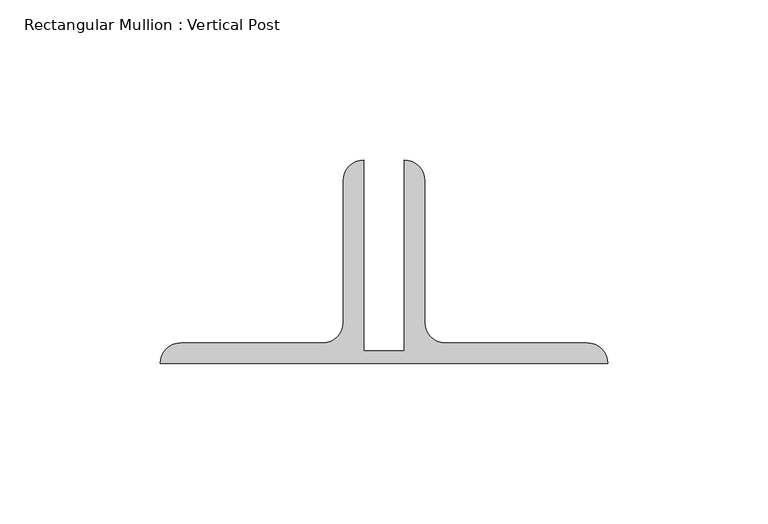
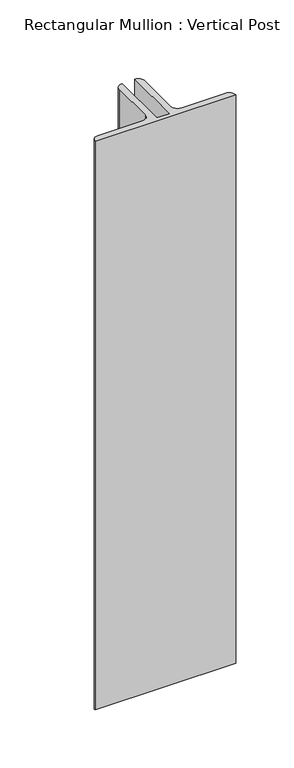
"""IFC4 building model written with IfcOpenShell, lengths in millimetres: member geometry, Rectangular Mullion : Vertical Post."""

from ifc_helpers import new_model, si_unit, point, frame, frame_2d, origin, place, context, project, spatial, polyline, circle_curve, trimmed, segment, composite_curve, outline, extrude, source, transform, mapped, element, save


def rectangular_mullion_vertical_post_30249c29(model_context):
    return source(origin(), model_context, "Body", "SweptSolid", [
        extrude(outline(composite_curve([segment(polyline([(-63.5, 22.9145205), (-63.5, 82.55)]), True, "CONTINUOUS"), segment(trimmed(circle_curve(frame_2d((-63.5, 76.2)), 6.35), [point((-63.5, 82.55))], [point((-57.15, 76.2))], False, "CARTESIAN"), True, "CONTINUOUS"), segment(polyline([(-57.15, 76.2), (-57.15, 31.75)]), True, "CONTINUOUS"), segment(trimmed(circle_curve(frame_2d((-50.8, 31.75)), 6.35), [point((-57.15, 31.75))], [point((-50.8, 25.4))], True, "CARTESIAN"), True, "CONTINUOUS"), segment(polyline([(-50.8, 25.4), (-6.35, 25.4)]), True, "CONTINUOUS"), segment(trimmed(circle_curve(frame_2d((-6.35, 19.05)), 6.35), [point((-6.35, 25.4))], [point((0.0, 19.05))], False, "CARTESIAN"), True, "CONTINUOUS"), segment(polyline([(0.0, 19.05), (-139.7, 19.05)]), True, "CONTINUOUS"), segment(trimmed(circle_curve(frame_2d((-133.35, 19.05)), 6.35), [point((-139.7, 19.05))], [point((-133.35, 25.4))], False, "CARTESIAN"), True, "CONTINUOUS"), segment(polyline([(-133.35, 25.4), (-88.9, 25.4)]), True, "CONTINUOUS"), segment(trimmed(circle_curve(frame_2d((-88.9, 31.75)), 6.35), [point((-88.9, 25.4))], [point((-82.55, 31.75))], True, "CARTESIAN"), True, "CONTINUOUS"), segment(polyline([(-82.55, 31.75), (-82.55, 76.2)]), True, "CONTINUOUS"), segment(trimmed(circle_curve(frame_2d((-76.2, 76.2)), 6.35), [point((-82.55, 76.2))], [point((-76.2, 82.55))], False, "CARTESIAN"), True, "CONTINUOUS"), segment(polyline([(-76.2, 82.55), (-76.2, 22.9145205), (-63.5, 22.9145205)]), True, "CONTINUOUS")], self_intersect=False)), frame((0.0, 0.0, -596.9), z_axis=(0.0, 0.0, 1.0), x_axis=(1.0, 0.0, 0.0)), (0.0, 0.0, 1.0), 596.9),
    ])


if __name__ == "__main__":
    model = new_model("IFC4")
    model_context = context("Model", 3, world=origin())
    ifc_project = project(units=[si_unit("LENGTHUNIT", "METRE", prefix="MILLI")], contexts=[model_context])
    site = spatial("IfcSite", under=ifc_project)
    building = spatial("IfcBuilding", under=site)
    placement = place(None, origin())
    rectangular_mullion_vertical_post_shape = rectangular_mullion_vertical_post_30249c29(model_context)
    element("IfcMember", 1, ObjectType="Rectangular Mullion : Vertical Post", at=placement, inside=building, context=model_context, shape_type="MappedRepresentation", body=[
        mapped(rectangular_mullion_vertical_post_shape, transform((0.0, 0.0, 0.0), x_axis=(1.0, 0.0, 0.0), y_axis=(0.0, 1.0, 0.0), z_axis=(0.0, 0.0, 1.0))),
    ])
    save(model, "model.ifc")

# Revit data of these elements
# Type "Rectangular Mullion : Vertical Post"
#   built-in parameter 1007351 = -0.0625 (stored number, unit not read)
#   built-in parameter 1007322 = 0.0126789 (stored number, unit not read)
#   built-in parameter 1007321 = 0.229167 (stored number, unit not read)
#   built-in parameter 1007320 = 0.229167 (stored number, unit not read)
# Element 1 (IfcMember, "Rectangular Mullion : Vertical Post")
#   Materials on its faces: "GATE POST: GALVANIZED ANGLES"
# Materials
#   "GATE POST: GALVANIZED ANGLES": class "Unassigned", colour RGB 211 211 211, transparency 0, Cost = 0
